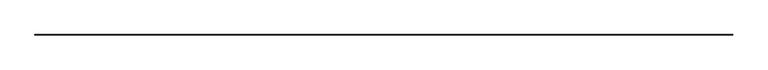
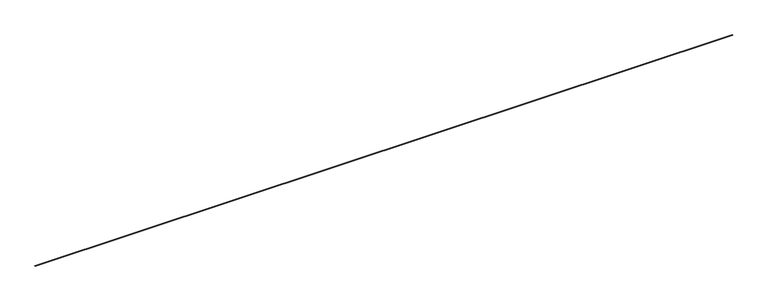
"""IFC4 building model written with IfcOpenShell, lengths in millimetres: proxy geometry, Inner panel:Inner panel:1:Inner panel:1 : Inner panel:Inner panel:300324:2:Inner panel:1:Inner panel:1 : Inner panel:Inner panel:300324:2 : Inner panel:Inner panel:1:Inner panel:1 : Inner panel:Inner panel:300324:300043:40 : Inner panel:Inner panel:1:Inner panel:1 : Inner panel:Inner panel:300324:2:Inner panel:1:Inner panel:1 : Inner panel:Inner panel:300324:2 : Inner panel:Inner panel:1:Inner panel:1 : Inner panel:Inner panel:300324:300043:308120."""

from ifc_helpers import new_model, si_unit, frame, origin, place, context, project, spatial, polyline, outline, extrude, source, transform, mapped, element, save


def generic_models_1fe2585a(model_context):
    return source(origin(), model_context, "Body", "SweptSolid", [
        extrude(outline(polyline([(-579097.5288841, 3907.730397), (-579099.1150078, 3945.7973671), (-579061.0480378, 3947.3834909), (-579059.461914, 3909.3165208), (-579097.5288841, 3907.730397)]), holes=[polyline([(-579095.2488312, 3910.2087154), (-579061.9402324, 3911.5965737), (-579063.3280907, 3944.9051725), (-579096.6366895, 3943.5173142), (-579095.2488312, 3910.2087154)])]), frame((579104.5117239, 0.0, 0.0), z_axis=(1.0, 0.0, 0.0), x_axis=(0.0, 1.0, 0.0)), (0.0, 0.0, 1.0), 88442.8),
    ])


if __name__ == "__main__":
    model = new_model("IFC4")
    model_context = context("Model", 3, world=origin())
    ifc_project = project(units=[si_unit("LENGTHUNIT", "METRE", prefix="MILLI")], contexts=[model_context])
    site = spatial("IfcSite", under=ifc_project)
    building = spatial("IfcBuilding", under=site)
    placement = place(None, origin())
    generic_models_shape = generic_models_1fe2585a(model_context)
    element("IfcBuildingElementProxy", 1, Name="Inner panel:Inner panel:1:Inner panel:1 : Inner panel:Inner panel:300324:2:Inner panel:1:Inner panel:1 : Inner panel:Inner panel:300324:2 : Inner panel:Inner panel:1:Inner panel:1 : Inner panel:Inner panel:300324:300043:40 : Inner panel:Inner panel:1:Inner panel:1 : Inner panel:Inner panel:300324:2:Inner panel:1:Inner panel:1 : Inner panel:Inner panel:300324:2 : Inner panel:Inner panel:1:Inner panel:1 : Inner panel:Inner panel:300324:300043:308120", ObjectType="Inner panel:Inner panel:1:Inner panel:1 : Inner panel:Inner panel:300324:2:Inner panel:1:Inner panel:1 : Inner panel:Inner panel:300324:2 : Inner panel:Inner panel:1:Inner panel:1 : Inner panel:Inner panel:300324:300043:40 : Inner panel:Inner panel:1:Inner panel:1 : Inner panel:Inner panel:300324:2:Inner panel:1:Inner panel:1 : Inner panel:Inner panel:300324:2 : Inner panel:Inner panel:1:Inner panel:1 : Inner panel:Inner panel:300324:300043:308120", at=placement, inside=building, context=model_context, shape_type="MappedRepresentation", body=[
        mapped(generic_models_shape, transform((0.0, 0.0, 0.0), x_axis=(1.0, 0.0, 0.0), y_axis=(0.0, 1.0, 0.0), z_axis=(0.0, 0.0, 1.0))),
    ])
    save(model, "model.ifc")

# Revit data of these elements
# Type "Inner panel:Inner panel:1:Inner panel:1 : Inner panel:Inner panel:300324:2:Inner panel:1:Inner panel:1 : Inner panel:Inner panel:300324:2 : Inner panel:Inner panel:1:Inner panel:1 : Inner panel:Inner panel:300324:300043:40 : Inner panel:Inner panel:1:Inner panel:1 : Inner panel:Inner panel:300324:2:Inner panel:1:Inner panel:1 : Inner panel:Inner panel:300324:2 : Inner panel:Inner panel:1:Inner panel:1 : Inner panel:Inner panel:300324:300043:308120"
#   NameOverride = "Inner panel:Inner panel:1:Inner panel:1 : Inner panel:Inner panel:300324:2:Inner panel:1:Inner panel:1 : Inner panel:Inner panel:300324:2 : Inner panel:Inner panel:1:Inner panel:1 : Inner panel:Inner panel:300324:300043:308120"
#   ObjectTypeOverride = "Inner panel:1:Inner panel:1 : Inner panel:Inner panel:300324:2 : Inner panel:Inner panel:1:Inner panel:1 : Inner panel:Inner panel:300324:300043"
#   Reference = "Inner panel"
#   Tag = "308120"
# Element 1 (IfcBuildingElementProxy, "Inner panel:Inner panel:1:Inner panel:1 : Inner panel:Inner panel:300324:2:Inner panel:1:Inner panel:1 : Inner panel:Inner panel:300324:2 : Inner panel:Inner panel:1:Inner panel:1 : Inner panel:Inner panel:300324:300043:40 : Inner panel:Inner panel:1:Inner panel:1 : Inner panel:Inner panel:300324:2:Inner panel:1:Inner panel:1 : Inner panel:Inner panel:300324:2 : Inner panel:Inner panel:1:Inner panel:1 : Inner panel:Inner panel:300324:300043:308120")
#   Materials on its faces: "1 1/2\" X 1 1/2\" x 1/8\" ALUM. TUBE (6061-T6) - (2) #16 WOOD SCREWS WITH 2.5\" EMBED AT EACH GLULAM - (1) SCREW AT ENDS"
# Materials
#   "1 1/2\" X 1 1/2\" x 1/8\" ALUM. TUBE (6061-T6) - (2) #16 WOOD SCREWS WITH 2.5\" EMBED AT EACH GLULAM - (1) SCREW AT ENDS": class "Unassigned", colour RGB 202 201 200, transparency 0, Cost = 0
